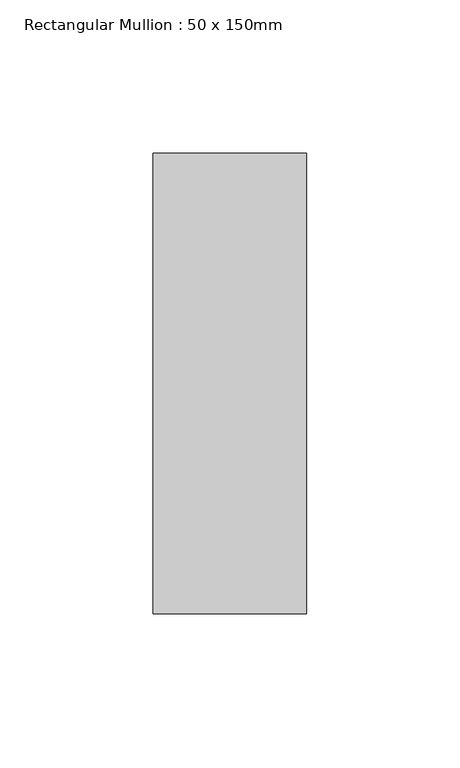
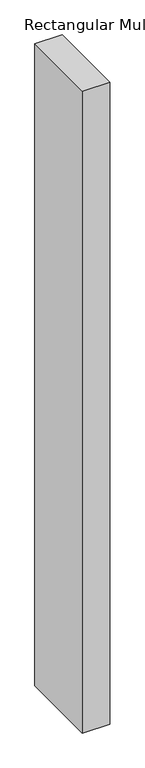
"""IFC4 building model written with IfcOpenShell, lengths in millimetres: member geometry, Rectangular Mullion : 50 x 150mm."""

import ifcopenshell
import ifcopenshell.guid

model = None  # the IFC model being written
_history = None  # IfcOwnerHistory: only IFC2X3 demands one
_inside = {}  # id of a spatial element -> (the spatial element, [elements in it])
_under = {}  # id of a project, library or spatial element -> (it, [spatial elements below it])
_declared = {}  # id of a project -> (the project, [libraries it declares])
_typed = {}  # id of a type object -> (the type object, [elements of that type])
_made_of = {}  # id of a material, layer set ... -> (it, [elements and type objects made of it])


def new_model(schema):
    """Start an empty IFC model of exactly this schema.

    Asked for "IFC4X3", IfcOpenShell would pick the latest addendum, in which some entities
    have other attributes; the version numbers below select the first issue.
    IFC2X3 requires an IfcOwnerHistory on every rooted entity: one is made here for all.
    """
    global model, _history
    if schema == "IFC4X3":
        model = ifcopenshell.file(schema_version=(4, 3, 0, 0))
    else:
        model = ifcopenshell.file(schema=schema)
    _inside.clear()
    _under.clear()
    _declared.clear()
    _typed.clear()
    _made_of.clear()
    _history = None
    if model.schema == "IFC2X3":
        org = make("IfcOrganization", Name="unknown")
        user = make(
            "IfcPersonAndOrganization",
            ThePerson=make("IfcPerson", FamilyName="unknown"),
            TheOrganization=org,
        )
        app = make(
            "IfcApplication",
            ApplicationDeveloper=org,
            Version="unknown",
            ApplicationFullName="unknown",
            ApplicationIdentifier="unknown",
        )
        _history = make(
            "IfcOwnerHistory",
            OwningUser=user,
            OwningApplication=app,
            ChangeAction="ADDED",
            CreationDate=0,
        )
    return model


def make(cls, **values):
    """One entity of the class cls with the attributes given. An attribute that is None is left unset."""
    return model.create_entity(
        cls, **{name: value for name, value in values.items() if value is not None}
    )


def rooted(cls, **values):
    """An entity with a GlobalId (a new one), such as an element, a storey or a relation."""
    return make(cls, GlobalId=ifcopenshell.guid.new(), OwnerHistory=_history, **values)


def si_unit(unit_type, name, prefix=None):
    """IfcSIUnit, for example si_unit("LENGTHUNIT", "METRE", prefix="MILLI")."""
    return make("IfcSIUnit", UnitType=unit_type, Prefix=prefix, Name=name)


def assignment(units):
    """IfcUnitAssignment: the units of a project."""
    return None if units is None else make("IfcUnitAssignment", Units=units)


def point(xyz):
    """IfcCartesianPoint."""
    return None if xyz is None else make("IfcCartesianPoint", Coordinates=xyz)


def direction(xyz):
    """IfcDirection."""
    return None if xyz is None else make("IfcDirection", DirectionRatios=xyz)


def frame(location, z_axis=None, x_axis=None):
    """IfcAxis2Placement3D, a coordinate frame: its origin and axes. An axis left out is left unset."""
    return make(
        "IfcAxis2Placement3D",
        Location=point(location),
        Axis=direction(z_axis),
        RefDirection=direction(x_axis),
    )


def origin():
    """The frame at (0, 0, 0) with its axes left unset."""
    return frame((0.0, 0.0, 0.0))


def place(relative_to, where):
    """IfcLocalPlacement: puts the frame where relative to a parent placement (None: the world)."""
    return make(
        "IfcLocalPlacement", PlacementRelTo=relative_to, RelativePlacement=where
    )


def context(
    kind, dimensions, precision=None, world=None, true_north=None, identifier=None
):
    """IfcGeometricRepresentationContext, for example the 3D "Model" context."""
    return make(
        "IfcGeometricRepresentationContext",
        ContextIdentifier=identifier,
        ContextType=kind,
        CoordinateSpaceDimension=dimensions,
        Precision=precision,
        WorldCoordinateSystem=world,
        TrueNorth=true_north,
    )


def project(units=None, contexts=None):
    """IfcProject with its units and contexts."""
    return rooted(
        "IfcProject",
        Name="project",
        RepresentationContexts=contexts,
        UnitsInContext=assignment(units),
    )


def spatial(cls, under=None, at=None, **own):
    """A site, building, storey or space (cls), placed at a placement, below another one or the project."""
    s = rooted(cls, ObjectPlacement=at, **own)
    if under is not None:
        _under.setdefault(under.id(), (under, []))[1].append(s)
    return s


def polyline(points):
    """IfcPolyline through the points."""
    return make("IfcPolyline", Points=[point(p) for p in points])


def outline(outer, holes=None, kind="AREA"):
    """IfcArbitraryClosedProfileDef: a profile drawn as a closed curve; with holes, ...WithVoids."""
    if holes is None:
        return make("IfcArbitraryClosedProfileDef", ProfileType=kind, OuterCurve=outer)
    return make(
        "IfcArbitraryProfileDefWithVoids",
        ProfileType=kind,
        OuterCurve=outer,
        InnerCurves=holes,
    )


def extrude(swept, where, along, depth):
    """IfcExtrudedAreaSolid: the profile swept, set in the frame where, extruded along a direction by depth."""
    return make(
        "IfcExtrudedAreaSolid",
        SweptArea=swept,
        Position=where,
        ExtrudedDirection=direction(along),
        Depth=depth,
    )


def shape(context_of_items, identifier, shape_type, items):
    """IfcShapeRepresentation: the items that make up one representation, for example the "Body"."""
    return make(
        "IfcShapeRepresentation",
        ContextOfItems=context_of_items,
        RepresentationIdentifier=identifier,
        RepresentationType=shape_type,
        Items=items,
    )


def source(mapping_origin, context_of_items, identifier, shape_type, items):
    """IfcRepresentationMap: a shape defined once, which mapped items show again and again."""
    return make(
        "IfcRepresentationMap",
        MappingOrigin=mapping_origin,
        MappedRepresentation=shape(context_of_items, identifier, shape_type, items),
    )


def transform(
    local_origin,
    x_axis=None,
    y_axis=None,
    z_axis=None,
    scale=None,
    scale2=None,
    scale3=None,
    uniform=True,
):
    """IfcCartesianTransformationOperator3D, or its non-uniform kind. x_axis, y_axis, z_axis: its Axis1, 2, 3."""
    if uniform:
        return make(
            "IfcCartesianTransformationOperator3D",
            Axis1=direction(x_axis),
            Axis2=direction(y_axis),
            LocalOrigin=point(local_origin),
            Scale=scale,
            Axis3=direction(z_axis),
        )
    return make(
        "IfcCartesianTransformationOperator3DnonUniform",
        Axis1=direction(x_axis),
        Axis2=direction(y_axis),
        LocalOrigin=point(local_origin),
        Scale=scale,
        Axis3=direction(z_axis),
        Scale2=scale2,
        Scale3=scale3,
    )


def mapped(mapping_source, mapping_target):
    """IfcMappedItem: shows the shape of a source again, moved by a transform."""
    return make(
        "IfcMappedItem", MappingSource=mapping_source, MappingTarget=mapping_target
    )


def made_of(thing, what):
    """Note that an element or type object is made of a material, layer set ...; save() writes the relation."""
    if what is not None:
        _made_of.setdefault(what.id(), (what, []))[1].append(thing)
    return thing


def element(
    cls,
    number,
    at=None,
    inside=None,
    cuts=None,
    type_object=None,
    material=None,
    context=None,
    identifier="Body",
    shape_type=None,
    held_by="IfcProductDefinitionShape",
    body=None,
    shapes=None,
    **own,
):
    """One element of the class cls, such as IfcWall. Its Tag is "e" and its number.

    at: its placement. inside: the storey or other place that contains it. cuts: it is an
    opening in that element (IfcRelVoidsElement). A single representation is given by context,
    identifier, shape_type and body (its items); several are given by shapes. held_by: the class
    of the entity that holds the representations. save() writes the other relations.
    """
    e = rooted(cls, Tag="e%d" % number, ObjectPlacement=at, **own)
    if body is not None:
        shapes = [shape(context, identifier, shape_type, body)]
    if shapes is not None:
        e.Representation = make(held_by, Representations=shapes)
    if inside is not None:
        _inside.setdefault(inside.id(), (inside, []))[1].append(e)
    if cuts is not None:
        rooted(
            "IfcRelVoidsElement", RelatingBuildingElement=cuts, RelatedOpeningElement=e
        )
    if type_object is not None:
        _typed.setdefault(type_object.id(), (type_object, []))[1].append(e)
    return made_of(e, material)


def aggregate(whole, parts):
    """IfcRelAggregates: a whole, such as a stair, and the parts it consists of."""
    return rooted("IfcRelAggregates", RelatingObject=whole, RelatedObjects=parts)


def save(model, path):
    """Write the relations noted so far, then the file.

    IfcRelAggregates (storeys below a building ...), IfcRelContainedInSpatialStructure (elements
    in a storey), IfcRelDefinesByType, IfcRelAssociatesMaterial and IfcRelDeclares: one each for
    every whole, place, type object, material and project.
    """
    for whole, parts in _under.values():
        aggregate(whole, parts)
    for where, things in _inside.values():
        rooted(
            "IfcRelContainedInSpatialStructure",
            RelatedElements=things,
            RelatingStructure=where,
        )
    for kind, things in _typed.values():
        rooted("IfcRelDefinesByType", RelatedObjects=things, RelatingType=kind)
    for what, things in _made_of.values():
        rooted("IfcRelAssociatesMaterial", RelatedObjects=things, RelatingMaterial=what)
    for by, libraries in _declared.values():
        rooted("IfcRelDeclares", RelatingContext=by, RelatedDefinitions=libraries)
    model.write(path)


def rectangular_mullion_50_x_150mm_49395e3f(model_context):
    return source(origin(), model_context, "Body", "SweptSolid", [
        extrude(outline(polyline([(0.0, 75.0), (0.0, -75.0), (-50.0, -75.0), (-50.0, 75.0), (0.0, 75.0)])), frame((0.0, 0.0, -1240.0000002), z_axis=(0.0, 0.0, 1.0), x_axis=(1.0, 0.0, 0.0)), (0.0, 0.0, 1.0), 1240.0000002),
    ])


if __name__ == "__main__":
    model = new_model("IFC4")
    model_context = context("Model", 3, world=origin())
    ifc_project = project(units=[si_unit("LENGTHUNIT", "METRE", prefix="MILLI")], contexts=[model_context])
    site = spatial("IfcSite", under=ifc_project)
    building = spatial("IfcBuilding", under=site)
    placement = place(None, origin())
    rectangular_mullion_50_x_150mm_shape = rectangular_mullion_50_x_150mm_49395e3f(model_context)
    element("IfcMember", 1, ObjectType="Rectangular Mullion : 50 x 150mm", at=placement, inside=building, context=model_context, shape_type="MappedRepresentation", body=[
        mapped(rectangular_mullion_50_x_150mm_shape, transform((0.0, 0.0, 0.0), x_axis=(1.0, 0.0, 0.0), y_axis=(0.0, 1.0, 0.0), z_axis=(0.0, 0.0, 1.0))),
    ])
    save(model, "model.ifc")

# Revit data of these elements
# Type "Rectangular Mullion : 50 x 150mm"
#   built-in parameter 1007304 = 0.492126 (stored number, unit not read)
#   built-in parameter 1007301 = 0.082021 (stored number, unit not read)
#   built-in parameter 1007300 = 0.082021 (stored number, unit not read)
# Element 1 (IfcMember, "Rectangular Mullion : 50 x 150mm")
#   Materials on its faces: "Aluminium"
# Materials
#   "Aluminium": class "Metal", colour RGB 247 247 247, transparency 0, Description = "Aluminium 6061", Cost = 0
